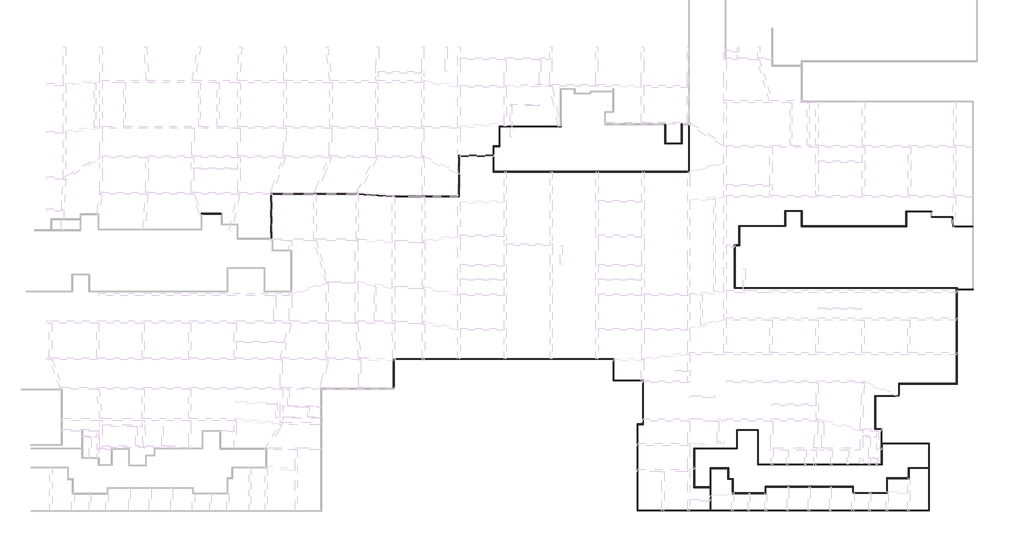
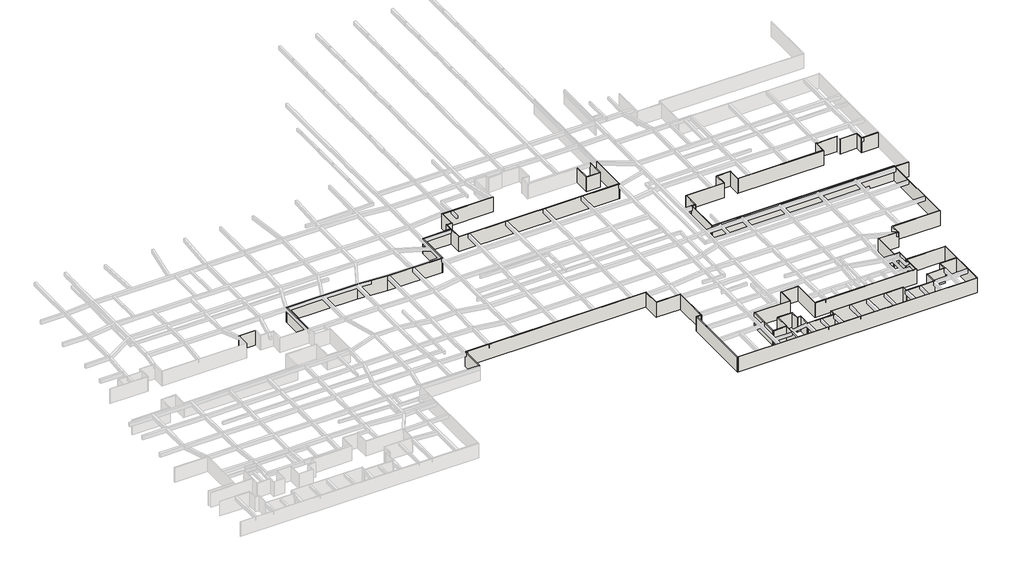
# One storey, part 2 of 16: 71 walls.
"""IFC4 building model written with IfcOpenShell, lengths in millimetres."""

from ifc_helpers import new_model, si_unit, origin, origin_with_axes, place, context, project, spatial, polyline, outline, extrude, faceted_brep, element, save

model = new_model("IFC4")

# Units and contexts
model_context = context("Model", 3, world=origin())
ifc_project = project(units=[si_unit("LENGTHUNIT", "METRE", prefix="MILLI")], contexts=[model_context])

# Site, building, storey
site = spatial("IfcSite", under=ifc_project)
building = spatial("IfcBuilding", under=site)
storey = spatial("IfcBuildingStorey", under=building, Name="户型图", Elevation=0.0)

# Walls
placement = place(None, origin())
element("IfcWall", 1, ObjectType="所有墙体", at=placement, inside=storey, context=model_context, shape_type="Brep", body=[
    faceted_brep([(130041.0654488, 81464.6119076, 0.0), (130041.0654488, 86623.7129117, 0.0), (130041.0654488, 86743.7129117, 0.0), (130041.0654488, 86743.7129117, 3300.0), (130041.0654488, 86623.7129117, 3300.0), (130041.0654488, 81464.6119076, 3300.0), (129921.0654488, 81464.6119076, 0.0), (129921.0654488, 81464.6119076, 3300.0), (129921.0654488, 86743.7129117, 3300.0), (129921.0654488, 86743.7129117, 0.0)], [[[0, 1, 2, 3, 4, 5]], [[6, 7, 8, 9]], [[2, 1, 0, 6, 9]], [[5, 4, 3, 8, 7]], [[0, 5, 7, 6]], [[3, 2, 9, 8]]]),
])
element("IfcWall", 2, ObjectType="所有墙体", at=placement, inside=storey, context=model_context, shape_type="Brep", body=[
    faceted_brep([(130041.0654488, 86623.7129117, 0.0), (168621.0654488, 86623.7129117, 0.0), (168741.0654488, 86623.7129117, 0.0), (168741.0654488, 86623.7129117, 3300.0), (168621.0654488, 86623.7129117, 3300.0), (130041.0654488, 86623.7129117, 3300.0), (130041.0654488, 86743.7129117, 0.0), (130041.0654488, 86743.7129117, 3300.0), (168741.0654488, 86743.7129117, 3300.0), (168741.0654488, 86743.7129117, 0.0)], [[[0, 1, 2, 3, 4, 5]], [[6, 7, 8, 9]], [[2, 1, 0, 6, 9]], [[5, 4, 3, 8, 7]], [[0, 5, 7, 6]], [[3, 2, 9, 8]]]),
])
element("IfcWall", 3, ObjectType="所有墙体", at=placement, inside=storey, context=model_context, shape_type="Brep", body=[
    faceted_brep([(168621.0654488, 86623.7129117, 0.0), (168621.0654488, 82792.1509701, 0.0), (168621.0654488, 82792.1509701, 3300.0), (168621.0654488, 86623.7129117, 3300.0), (168741.0654488, 86623.7129117, 0.0), (168741.0654488, 86623.7129117, 3300.0), (168741.0654488, 82912.1509701, 3300.0), (168741.0654488, 82792.1509701, 3300.0), (168741.0654488, 82792.1509701, 0.0), (168741.0654488, 82912.1509701, 0.0)], [[[0, 1, 2, 3]], [[4, 5, 6, 7, 8, 9]], [[1, 0, 4, 9, 8]], [[3, 2, 7, 6, 5]], [[0, 3, 5, 4]], [[2, 1, 8, 7]]]),
])
element("IfcWall", 4, ObjectType="所有墙体", at=placement, inside=storey, context=model_context, shape_type="Brep", body=[
    faceted_brep([(168741.0654488, 82792.1509701, 0.0), (173812.0751369, 82792.1509701, 0.0), (173932.0751369, 82792.1509701, 0.0), (173932.0751369, 82792.1509701, 3300.0), (173812.0751369, 82792.1509701, 3300.0), (168741.0654488, 82792.1509701, 3300.0), (168741.0654488, 82912.1509701, 0.0), (168741.0654488, 82912.1509701, 3300.0), (173932.0751369, 82912.1509701, 3300.0), (173932.0751369, 82912.1509701, 0.0)], [[[0, 1, 2, 3, 4, 5]], [[6, 7, 8, 9]], [[2, 1, 0, 6, 9]], [[5, 4, 3, 8, 7]], [[0, 5, 7, 6]], [[3, 2, 9, 8]]]),
])
element("IfcWall", 5, ObjectType="所有墙体", at=placement, inside=storey, context=model_context, shape_type="Brep", body=[
    faceted_brep([(173812.0751369, 82792.1509701, 0.0), (173812.0751369, 75212.1509701, 0.0), (173812.0751369, 75092.1509701, 0.0), (173812.0751369, 75092.1509701, 3300.0), (173812.0751369, 75212.1509701, 3300.0), (173812.0751369, 82792.1509701, 3300.0), (173932.0751369, 82792.1509701, 0.0), (173932.0751369, 82792.1509701, 3300.0), (173932.0751369, 75092.1509701, 3300.0), (173932.0751369, 75092.1509701, 0.0)], [[[0, 1, 2, 3, 4, 5]], [[6, 7, 8, 9]], [[2, 1, 0, 6, 9]], [[5, 4, 3, 8, 7]], [[0, 5, 7, 6]], [[3, 2, 9, 8]]]),
])
element("IfcWall", 6, ObjectType="所有墙体", at=placement, inside=storey, context=model_context, shape_type="Brep", body=[
    faceted_brep([(173812.0751369, 75212.1509701, 0.0), (172837.1171537, 75212.1509701, 0.0), (172837.1171537, 75212.1509701, 3300.0), (173812.0751369, 75212.1509701, 3300.0), (173812.0751369, 75092.1509701, 0.0), (173812.0751369, 75092.1509701, 3300.0), (172957.1171537, 75092.1509701, 3300.0), (172837.1171537, 75092.1509701, 3300.0), (172837.1171537, 75092.1509701, 0.0), (172957.1171537, 75092.1509701, 0.0)], [[[0, 1, 2, 3]], [[4, 5, 6, 7, 8, 9]], [[1, 0, 4, 9, 8]], [[3, 2, 7, 6, 5]], [[0, 3, 5, 4]], [[2, 1, 8, 7]]]),
])
element("IfcWall", 7, ObjectType="所有墙体", at=placement, inside=storey, context=model_context, shape_type="Brep", body=[
    faceted_brep([(172837.1171537, 75092.1509701, 0.0), (172837.1171537, 59892.1509701, 0.0), (172837.1171537, 59892.1509701, 3300.0), (172837.1171537, 75092.1509701, 3300.0), (172957.1171537, 75092.1509701, 0.0), (172957.1171537, 75092.1509701, 3300.0), (172957.1171537, 60012.1509701, 3300.0), (172957.1171537, 59892.1509701, 3300.0), (172957.1171537, 59892.1509701, 0.0), (172957.1171537, 60012.1509701, 0.0)], [[[0, 1, 2, 3]], [[4, 5, 6, 7, 8, 9]], [[1, 0, 4, 9, 8]], [[3, 2, 7, 6, 5]], [[0, 3, 5, 4]], [[2, 1, 8, 7]]]),
])
element("IfcWall", 8, ObjectType="所有墙体", at=placement, inside=storey, context=model_context, shape_type="Brep", body=[
    faceted_brep([(172957.1171537, 59892.1509701, 0.0), (224357.1171537, 59892.1509701, 0.0), (224357.1171537, 59892.1509701, 3300.0), (172957.1171537, 59892.1509701, 3300.0), (172957.1171537, 60012.1509701, 0.0), (172957.1171537, 60012.1509701, 3300.0), (185686.7118802, 60012.1509701, 3300.0), (185806.7118802, 60012.1509701, 3300.0), (224237.1171537, 60012.1509701, 3300.0), (224357.1171537, 60012.1509701, 3300.0), (224357.1171537, 60012.1509701, 0.0), (224237.1171537, 60012.1509701, 0.0), (185806.7118802, 60012.1509701, 0.0), (185686.7118802, 60012.1509701, 0.0)], [[[0, 1, 2, 3]], [[4, 5, 6, 7, 8, 9, 10, 11, 12, 13]], [[1, 0, 4, 13, 12, 11, 10]], [[3, 2, 9, 8, 7, 6, 5]], [[0, 3, 5, 4]], [[2, 1, 10, 9]]]),
])
element("IfcWall", 9, ObjectType="所有墙体", at=placement, inside=storey, context=model_context, shape_type="Brep", body=[
    faceted_brep([(224357.1171537, 60012.1509701, 0.0), (224357.1171537, 71812.1509701, 0.0), (224357.1171537, 71812.1509701, 3300.0), (224357.1171537, 60012.1509701, 3300.0), (224237.1171537, 60012.1509701, 0.0), (224237.1171537, 60012.1509701, 3300.0), (224237.1171537, 67402.3902279, 3300.0), (224237.1171537, 67522.3902279, 3300.0), (224237.1171537, 71692.1509701, 3300.0), (224237.1171537, 71812.1509701, 3300.0), (224237.1171537, 71812.1509701, 0.0), (224237.1171537, 71692.1509701, 0.0), (224237.1171537, 67522.3902279, 0.0), (224237.1171537, 67402.3902279, 0.0)], [[[0, 1, 2, 3]], [[4, 5, 6, 7, 8, 9, 10, 11, 12, 13]], [[1, 0, 4, 13, 12, 11, 10]], [[3, 2, 9, 8, 7, 6, 5]], [[0, 3, 5, 4]], [[2, 1, 10, 9]]]),
])
element("IfcWall", 10, ObjectType="所有墙体", at=placement, inside=storey, context=model_context, shape_type="Brep", body=[
    faceted_brep([(224237.1171537, 71812.1509701, 0.0), (215957.1171537, 71812.1509701, 0.0), (215837.1171537, 71812.1509701, 0.0), (215837.1171537, 71812.1509701, 3300.0), (215957.1171537, 71812.1509701, 3300.0), (224237.1171537, 71812.1509701, 3300.0), (224237.1171537, 71692.1509701, 0.0), (224237.1171537, 71692.1509701, 3300.0), (216006.7104154, 71692.1509701, 3300.0), (215886.7104154, 71692.1509701, 3300.0), (215837.1171537, 71692.1509701, 3300.0), (215837.1171537, 71692.1509701, 0.0), (215886.7104154, 71692.1509701, 0.0), (216006.7104154, 71692.1509701, 0.0)], [[[0, 1, 2, 3, 4, 5]], [[6, 7, 8, 9, 10, 11, 12, 13]], [[2, 1, 0, 6, 13, 12, 11]], [[5, 4, 3, 10, 9, 8, 7]], [[0, 5, 7, 6]], [[3, 2, 11, 10]]]),
])
element("IfcWall", 11, ObjectType="所有墙体", at=placement, inside=storey, context=model_context, shape_type="Brep", body=[
    faceted_brep([(215957.1171537, 71812.1509701, 0.0), (215957.1171537, 74372.3072201, 0.0), (215957.1171537, 74372.3072201, 3300.0), (215957.1171537, 71812.1509701, 3300.0), (215837.1171537, 71812.1509701, 0.0), (215837.1171537, 71812.1509701, 3300.0), (215837.1171537, 74252.3072201, 3300.0), (215837.1171537, 74372.3072201, 3300.0), (215837.1171537, 74372.3072201, 0.0), (215837.1171537, 74252.3072201, 0.0)], [[[0, 1, 2, 3]], [[4, 5, 6, 7, 8, 9]], [[1, 0, 4, 9, 8]], [[3, 2, 7, 6, 5]], [[0, 3, 5, 4]], [[2, 1, 8, 7]]]),
])
element("IfcWall", 12, ObjectType="所有墙体", at=placement, inside=storey, context=model_context, shape_type="Brep", body=[
    faceted_brep([(215837.1171537, 74372.3072201, 0.0), (214857.1171537, 74372.3072201, 0.0), (214737.1171537, 74372.3072201, 0.0), (214737.1171537, 74372.3072201, 3300.0), (214857.1171537, 74372.3072201, 3300.0), (215837.1171537, 74372.3072201, 3300.0), (215837.1171537, 74252.3072201, 0.0), (215837.1171537, 74252.3072201, 3300.0), (214737.1171537, 74252.3072201, 3300.0), (214737.1171537, 74252.3072201, 0.0)], [[[0, 1, 2, 3, 4, 5]], [[6, 7, 8, 9]], [[2, 1, 0, 6, 9]], [[5, 4, 3, 8, 7]], [[0, 5, 7, 6]], [[3, 2, 9, 8]]]),
])
element("IfcWall", 13, ObjectType="所有墙体", at=placement, inside=storey, context=model_context, shape_type="Brep", body=[
    faceted_brep([(214857.1171537, 74372.3072201, 0.0), (214857.1171537, 80052.3072201, 0.0), (214857.1171537, 80172.3072201, 0.0), (214857.1171537, 80172.3072201, 3300.0), (214857.1171537, 80052.3072201, 3300.0), (214857.1171537, 74372.3072201, 3300.0), (214737.1171537, 74372.3072201, 0.0), (214737.1171537, 74372.3072201, 3300.0), (214737.1171537, 80172.3072201, 3300.0), (214737.1171537, 80172.3072201, 0.0)], [[[0, 1, 2, 3, 4, 5]], [[6, 7, 8, 9]], [[2, 1, 0, 6, 9]], [[5, 4, 3, 8, 7]], [[0, 5, 7, 6]], [[3, 2, 9, 8]]]),
])
element("IfcWall", 14, ObjectType="所有墙体", at=placement, inside=storey, context=model_context, shape_type="Brep", body=[
    faceted_brep([(214857.1171537, 80052.3072201, 0.0), (219065.7473941, 80052.3072201, 0.0), (219065.7473941, 80052.3072201, 3300.0), (214857.1171537, 80052.3072201, 3300.0), (214857.1171537, 80172.3072201, 0.0), (214857.1171537, 80172.3072201, 3300.0), (218945.7473941, 80172.3072201, 3300.0), (219065.7473941, 80172.3072201, 3300.0), (219065.7473941, 80172.3072201, 0.0), (218945.7473941, 80172.3072201, 0.0)], [[[0, 1, 2, 3]], [[4, 5, 6, 7, 8, 9]], [[1, 0, 4, 9, 8]], [[3, 2, 7, 6, 5]], [[0, 3, 5, 4]], [[2, 1, 8, 7]]]),
])
element("IfcWall", 15, ObjectType="所有墙体", at=placement, inside=storey, context=model_context, shape_type="Brep", body=[
    faceted_brep([(219065.7473941, 80172.3072201, 0.0), (219065.7473941, 82242.2134701, 0.0), (219065.7473941, 82362.2134701, 0.0), (219065.7473941, 82362.2134701, 3300.0), (219065.7473941, 82242.2134701, 3300.0), (219065.7473941, 80172.3072201, 3300.0), (218945.7473941, 80172.3072201, 0.0), (218945.7473941, 80172.3072201, 3300.0), (218945.7473941, 82362.2134701, 3300.0), (218945.7473941, 82362.2134701, 0.0)], [[[0, 1, 2, 3, 4, 5]], [[6, 7, 8, 9]], [[2, 1, 0, 6, 9]], [[5, 4, 3, 8, 7]], [[0, 5, 7, 6]], [[3, 2, 9, 8]]]),
])
element("IfcWall", 16, ObjectType="所有墙体", at=placement, inside=storey, context=model_context, shape_type="Brep", body=[
    faceted_brep([(219065.7473941, 82242.2134701, 0.0), (229226.2421537, 82242.2134701, 0.0), (229226.2421537, 82242.2134701, 3300.0), (219065.7473941, 82242.2134701, 3300.0), (219065.7473941, 82362.2134701, 0.0), (219065.7473941, 82362.2134701, 3300.0), (229106.2421537, 82362.2134701, 3300.0), (229226.2421537, 82362.2134701, 3300.0), (229226.2421537, 82362.2134701, 0.0), (229106.2421537, 82362.2134701, 0.0)], [[[0, 1, 2, 3]], [[4, 5, 6, 7, 8, 9]], [[1, 0, 4, 9, 8]], [[3, 2, 7, 6, 5]], [[0, 3, 5, 4]], [[2, 1, 8, 7]]]),
])
element("IfcWall", 17, ObjectType="所有墙体", at=placement, inside=storey, context=model_context, shape_type="Brep", body=[
    faceted_brep([(229226.2421537, 82362.2134701, 0.0), (229226.2421537, 98851.3072201, 0.0), (229226.2421537, 98971.3072201, 0.0), (229226.2421537, 99221.2967221, 0.0), (229226.2421537, 99221.2967221, 3300.0), (229226.2421537, 98971.3072201, 3300.0), (229226.2421537, 98851.3072201, 3300.0), (229226.2421537, 82362.2134701, 3300.0), (229106.2421537, 82362.2134701, 0.0), (229106.2421537, 82362.2134701, 3300.0), (229106.2421537, 99101.2967221, 3300.0), (229106.2421537, 99221.2967221, 3300.0), (229106.2421537, 99221.2967221, 0.0), (229106.2421537, 99101.2967221, 0.0)], [[[0, 1, 2, 3, 4, 5, 6, 7]], [[8, 9, 10, 11, 12, 13]], [[3, 2, 1, 0, 8, 13, 12]], [[7, 6, 5, 4, 11, 10, 9]], [[0, 7, 9, 8]], [[4, 3, 12, 11]]]),
])
element("IfcWall", 18, ObjectType="所有墙体", at=placement, inside=storey, context=model_context, shape_type="Brep", body=[
    faceted_brep([(229226.2421537, 98851.3072201, 0.0), (232107.9308744, 98851.3072201, 0.0), (232107.9308744, 98851.3072201, 3300.0), (229226.2421537, 98851.3072201, 3300.0), (229226.2421537, 98971.3072201, 0.0), (229226.2421537, 98971.3072201, 3300.0), (231987.9308744, 98971.3072201, 3300.0), (232107.9308744, 98971.3072201, 3300.0), (232107.9308744, 98971.3072201, 0.0), (231987.9308744, 98971.3072201, 0.0)], [[[0, 1, 2, 3]], [[4, 5, 6, 7, 8, 9]], [[1, 0, 4, 9, 8]], [[3, 2, 7, 6, 5]], [[2, 1, 8, 7]], [[0, 3, 5, 4]]]),
])
element("IfcWall", 19, ObjectType="所有墙体", at=placement, inside=storey, context=model_context, shape_type="Brep", body=[
    faceted_brep([(99612.3510404, 112314.5259701, 0.0), (96012.3510404, 112314.5259701, 0.0), (96012.3510404, 112314.5259701, 3300.0), (99612.3510404, 112314.5259701, 3300.0), (99612.3510404, 112194.5259701, 0.0), (99612.3510404, 112194.5259701, 3300.0), (96132.3510404, 112194.5259701, 3300.0), (96012.3510404, 112194.5259701, 3300.0), (96012.3510404, 112194.5259701, 0.0), (96132.3510404, 112194.5259701, 0.0)], [[[0, 1, 2, 3]], [[4, 5, 6, 7, 8, 9]], [[1, 0, 4, 9, 8]], [[3, 2, 7, 6, 5]], [[0, 3, 5, 4]], [[2, 1, 8, 7]]]),
])
element("IfcWall", 20, ObjectType="所有墙体", at=placement, inside=storey, context=model_context, shape_type="Brep", body=[
    faceted_brep([(177743.2890287, 127952.5884701, 0.0), (177743.2890287, 124552.5884701, 0.0), (177743.2890287, 124552.5884701, 3300.0), (177743.2890287, 127952.5884701, 3300.0), (177863.2890287, 127952.5884701, 0.0), (177863.2890287, 127952.5884701, 3300.0), (177863.2890287, 124672.5884701, 3300.0), (177863.2890287, 124552.5884701, 3300.0), (177863.2890287, 124552.5884701, 0.0), (177863.2890287, 124672.5884701, 0.0)], [[[0, 1, 2, 3]], [[4, 5, 6, 7, 8, 9]], [[1, 0, 4, 9, 8]], [[3, 2, 7, 6, 5]], [[0, 3, 5, 4]], [[2, 1, 8, 7]]]),
])
element("IfcWall", 21, ObjectType="所有墙体", at=placement, inside=storey, context=model_context, shape_type="Brep", body=[
    faceted_brep([(177863.2890287, 124552.5884701, 0.0), (180763.3460986, 124552.5884701, 0.0), (180763.3460986, 124552.5884701, 3300.0), (177863.2890287, 124552.5884701, 3300.0), (177863.2890287, 124672.5884701, 0.0), (177863.2890287, 124672.5884701, 3300.0), (180643.3460986, 124672.5884701, 3300.0), (180763.3460986, 124672.5884701, 3300.0), (180763.3460986, 124672.5884701, 0.0), (180643.3460986, 124672.5884701, 0.0)], [[[0, 1, 2, 3]], [[4, 5, 6, 7, 8, 9]], [[1, 0, 4, 9, 8]], [[3, 2, 7, 6, 5]], [[0, 3, 5, 4]], [[2, 1, 8, 7]]]),
])
element("IfcWall", 22, ObjectType="所有墙体", at=placement, inside=storey, context=model_context, shape_type="Brep", body=[
    faceted_brep([(180763.3460986, 124672.5884701, 0.0), (180763.3460986, 127952.5884701, 0.0), (180763.3460986, 128072.5884701, 0.0), (180763.3460986, 128072.5884701, 3300.0), (180763.3460986, 127952.5884701, 3300.0), (180763.3460986, 124672.5884701, 3300.0), (180643.3460986, 124672.5884701, 0.0), (180643.3460986, 124672.5884701, 3300.0), (180643.3460986, 128072.5884701, 3300.0), (180643.3460986, 128072.5884701, 0.0)], [[[0, 1, 2, 3, 4, 5]], [[6, 7, 8, 9]], [[2, 1, 0, 6, 9]], [[5, 4, 3, 8, 7]], [[0, 5, 7, 6]], [[3, 2, 9, 8]]]),
])
element("IfcWall", 23, ObjectType="所有墙体", at=placement, inside=storey, context=model_context, shape_type="Brep", body=[
    faceted_brep([(181897.7367524, 127952.5884701, 0.0), (181897.7367524, 119698.0259701, 0.0), (181897.7367524, 119578.0259701, 0.0), (181897.7367524, 119578.0259701, 3300.0), (181897.7367524, 119698.0259701, 3300.0), (181897.7367524, 127952.5884701, 3300.0), (182017.7367524, 127952.5884701, 0.0), (182017.7367524, 127952.5884701, 3300.0), (182017.7367524, 119578.0259701, 3300.0), (182017.7367524, 119578.0259701, 0.0)], [[[0, 1, 2, 3, 4, 5]], [[6, 7, 8, 9]], [[2, 1, 0, 6, 9]], [[5, 4, 3, 8, 7]], [[3, 2, 9, 8]], [[0, 5, 7, 6]]]),
])
element("IfcWall", 24, ObjectType="所有墙体", at=placement, inside=storey, context=model_context, shape_type="Brep", body=[
    faceted_brep([(181897.7367524, 119698.0259701, 0.0), (147617.7367524, 119698.0259701, 0.0), (147497.7367524, 119698.0259701, 0.0), (147497.7367524, 119698.0259701, 3300.0), (147617.7367524, 119698.0259701, 3300.0), (181897.7367524, 119698.0259701, 3300.0), (181897.7367524, 119578.0259701, 0.0), (181897.7367524, 119578.0259701, 3300.0), (147497.7367524, 119578.0259701, 3300.0), (147497.7367524, 119578.0259701, 0.0)], [[[0, 1, 2, 3, 4, 5]], [[6, 7, 8, 9]], [[2, 1, 0, 6, 9]], [[5, 4, 3, 8, 7]], [[0, 5, 7, 6]], [[3, 2, 9, 8]]]),
])
element("IfcWall", 25, ObjectType="所有墙体", at=placement, inside=storey, context=model_context, shape_type="Brep", body=[
    faceted_brep([(147617.7367524, 119698.0259701, 0.0), (147617.7367524, 124078.0259701, 0.0), (147617.7367524, 124198.0259701, 0.0), (147617.7367524, 124198.0259701, 3300.0), (147617.7367524, 124078.0259701, 3300.0), (147617.7367524, 119698.0259701, 3300.0), (147497.7367524, 119698.0259701, 0.0), (147497.7367524, 119698.0259701, 3300.0), (147497.7367524, 122418.0259701, 3300.0), (147497.7367524, 122538.0259701, 3300.0), (147497.7367524, 124198.0259701, 3300.0), (147497.7367524, 124198.0259701, 0.0), (147497.7367524, 122538.0259701, 0.0), (147497.7367524, 122418.0259701, 0.0)], [[[0, 1, 2, 3, 4, 5]], [[6, 7, 8, 9, 10, 11, 12, 13]], [[2, 1, 0, 6, 13, 12, 11]], [[5, 4, 3, 10, 9, 8, 7]], [[0, 5, 7, 6]], [[3, 2, 11, 10]]]),
])
element("IfcWall", 26, ObjectType="所有墙体", at=placement, inside=storey, context=model_context, shape_type="Brep", body=[
    faceted_brep([(147617.7367524, 124078.0259701, 0.0), (148663.2890287, 124078.0259701, 0.0), (148663.2890287, 124078.0259701, 3300.0), (147617.7367524, 124078.0259701, 3300.0), (147617.7367524, 124198.0259701, 0.0), (147617.7367524, 124198.0259701, 3300.0), (148543.2890287, 124198.0259701, 3300.0), (148663.2890287, 124198.0259701, 3300.0), (148663.2890287, 124198.0259701, 0.0), (148543.2890287, 124198.0259701, 0.0)], [[[0, 1, 2, 3]], [[4, 5, 6, 7, 8, 9]], [[1, 0, 4, 9, 8]], [[3, 2, 7, 6, 5]], [[0, 3, 5, 4]], [[2, 1, 8, 7]]]),
])
element("IfcWall", 27, ObjectType="所有墙体", at=placement, inside=storey, context=model_context, shape_type="Brep", body=[
    faceted_brep([(148663.2890287, 124198.0259701, 0.0), (148663.2890287, 127578.0259701, 0.0), (148663.2890287, 127698.0259701, 0.0), (148663.2890287, 127698.0259701, 3300.0), (148663.2890287, 127578.0259701, 3300.0), (148663.2890287, 124198.0259701, 3300.0), (148543.2890287, 124198.0259701, 0.0), (148543.2890287, 124198.0259701, 3300.0), (148543.2890287, 127698.0259701, 3300.0), (148543.2890287, 127698.0259701, 0.0)], [[[0, 1, 2, 3, 4, 5]], [[6, 7, 8, 9]], [[2, 1, 0, 6, 9]], [[5, 4, 3, 8, 7]], [[0, 5, 7, 6]], [[3, 2, 9, 8]]]),
])
element("IfcWall", 28, ObjectType="所有墙体", at=placement, inside=storey, context=model_context, shape_type="Brep", body=[
    faceted_brep([(148663.2890287, 127578.0259701, 0.0), (159463.2890287, 127578.0259701, 0.0), (159463.2890287, 127578.0259701, 3300.0), (148663.2890287, 127578.0259701, 3300.0), (148663.2890287, 127698.0259701, 0.0), (148663.2890287, 127698.0259701, 3300.0), (159343.2890287, 127698.0259701, 3300.0), (159463.2890287, 127698.0259701, 3300.0), (159463.2890287, 127698.0259701, 0.0), (159343.2890287, 127698.0259701, 0.0)], [[[0, 1, 2, 3]], [[4, 5, 6, 7, 8, 9]], [[1, 0, 4, 9, 8]], [[3, 2, 7, 6, 5]], [[0, 3, 5, 4]], [[2, 1, 8, 7]]]),
])
element("IfcWall", 29, ObjectType="所有墙体", at=placement, inside=storey, context=model_context, shape_type="Brep", body=[
    faceted_brep([(199007.9283109, 110171.2134701, 0.0), (198887.9283109, 110171.2134701, 0.0), (190787.9283109, 110171.2134701, 0.0), (190787.9283109, 110171.2134701, 3300.0), (198887.9283109, 110171.2134701, 3300.0), (199007.9283109, 110171.2134701, 3300.0), (199007.9283109, 110051.2134701, 0.0), (199007.9283109, 110051.2134701, 3300.0), (190907.9283109, 110051.2134701, 3300.0), (190787.9283109, 110051.2134701, 3300.0), (190787.9283109, 110051.2134701, 0.0), (190907.9283109, 110051.2134701, 0.0)], [[[0, 1, 2, 3, 4, 5]], [[6, 7, 8, 9, 10, 11]], [[2, 1, 0, 6, 11, 10]], [[5, 4, 3, 9, 8, 7]], [[3, 2, 10, 9]], [[0, 5, 7, 6]]]),
])
element("IfcWall", 30, ObjectType="所有墙体", at=placement, inside=storey, context=model_context, shape_type="Brep", body=[
    faceted_brep([(190787.9283109, 110051.2134701, 0.0), (190787.9283109, 106771.2090896, 0.0), (190787.9283109, 106651.2090896, 0.0), (190787.9283109, 106651.2090896, 3300.0), (190787.9283109, 106771.2090896, 3300.0), (190787.9283109, 110051.2134701, 3300.0), (190907.9283109, 110051.2134701, 0.0), (190907.9283109, 110051.2134701, 3300.0), (190907.9283109, 106651.2090896, 3300.0), (190907.9283109, 106651.2090896, 0.0)], [[[0, 1, 2, 3, 4, 5]], [[6, 7, 8, 9]], [[2, 1, 0, 6, 9]], [[5, 4, 3, 8, 7]], [[0, 5, 7, 6]], [[3, 2, 9, 8]]]),
])
element("IfcWall", 31, ObjectType="所有墙体", at=placement, inside=storey, context=model_context, shape_type="Brep", body=[
    faceted_brep([(190787.9283109, 106771.2090896, 0.0), (189987.9283109, 106771.2090896, 0.0), (189987.9283109, 106771.2090896, 3300.0), (190787.9283109, 106771.2090896, 3300.0), (190787.9283109, 106651.2090896, 0.0), (190787.9283109, 106651.2090896, 3300.0), (190107.9283109, 106651.2090896, 3300.0), (189987.9283109, 106651.2090896, 3300.0), (189987.9283109, 106651.2090896, 0.0), (190107.9283109, 106651.2090896, 0.0)], [[[0, 1, 2, 3]], [[4, 5, 6, 7, 8, 9]], [[1, 0, 4, 9, 8]], [[3, 2, 7, 6, 5]], [[0, 3, 5, 4]], [[2, 1, 8, 7]]]),
])
element("IfcWall", 32, ObjectType="所有墙体", at=placement, inside=storey, context=model_context, shape_type="Brep", body=[
    faceted_brep([(189987.9283109, 106651.2090896, 0.0), (189987.9283109, 99101.2967221, 0.0), (189987.9283109, 99101.2967221, 3300.0), (189987.9283109, 106651.2090896, 3300.0), (190107.9283109, 106651.2090896, 0.0), (190107.9283109, 106651.2090896, 3300.0), (190107.9283109, 99221.2967221, 3300.0), (190107.9283109, 99101.2967221, 3300.0), (190107.9283109, 99101.2967221, 0.0), (190107.9283109, 99221.2967221, 0.0)], [[[0, 1, 2, 3]], [[4, 5, 6, 7, 8, 9]], [[1, 0, 4, 9, 8]], [[3, 2, 7, 6, 5]], [[0, 3, 5, 4]], [[2, 1, 8, 7]]]),
])
element("IfcWall", 33, ObjectType="所有墙体", at=placement, inside=storey, context=model_context, shape_type="SweptSolid", body=[
    extrude(outline(polyline([(190107.9283109, 99221.2967221), (229106.2421537, 99221.2967221), (229106.2421537, 99101.2967221), (190107.9283109, 99101.2967221), (190107.9283109, 99221.2967221)])), origin_with_axes(), (0.0, 0.0, 1.0), 3300.0),
])
element("IfcWall", 34, ObjectType="所有墙体", at=placement, inside=storey, context=model_context, shape_type="Brep", body=[
    faceted_brep([(199007.9283109, 110171.2134701, 0.0), (199007.9283109, 112701.2124935, 0.0), (199007.9283109, 112821.2124935, 0.0), (199007.9283109, 112821.2124935, 3300.0), (199007.9283109, 112701.2124935, 3300.0), (199007.9283109, 110171.2134701, 3300.0), (198887.9283109, 110171.2134701, 0.0), (198887.9283109, 110171.2134701, 3300.0), (198887.9283109, 112821.2124935, 3300.0), (198887.9283109, 112821.2124935, 0.0)], [[[0, 1, 2, 3, 4, 5]], [[6, 7, 8, 9]], [[2, 1, 0, 6, 9]], [[5, 4, 3, 8, 7]], [[0, 5, 7, 6]], [[3, 2, 9, 8]]]),
])
element("IfcWall", 35, ObjectType="所有墙体", at=placement, inside=storey, context=model_context, shape_type="Brep", body=[
    faceted_brep([(199007.9283109, 112701.2124935, 0.0), (201787.9283109, 112701.2124935, 0.0), (201907.9283109, 112701.2124935, 0.0), (201907.9283109, 112701.2124935, 3300.0), (201787.9283109, 112701.2124935, 3300.0), (199007.9283109, 112701.2124935, 3300.0), (199007.9283109, 112821.2124935, 0.0), (199007.9283109, 112821.2124935, 3300.0), (201907.9283109, 112821.2124935, 3300.0), (201907.9283109, 112821.2124935, 0.0)], [[[0, 1, 2, 3, 4, 5]], [[6, 7, 8, 9]], [[2, 1, 0, 6, 9]], [[5, 4, 3, 8, 7]], [[0, 5, 7, 6]], [[3, 2, 9, 8]]]),
])
element("IfcWall", 36, ObjectType="所有墙体", at=placement, inside=storey, context=model_context, shape_type="Brep", body=[
    faceted_brep([(201787.9283109, 112701.2124935, 0.0), (201787.9283109, 110001.2124935, 0.0), (201787.9283109, 110001.2124935, 3300.0), (201787.9283109, 112701.2124935, 3300.0), (201907.9283109, 112701.2124935, 0.0), (201907.9283109, 112701.2124935, 3300.0), (201907.9283109, 110121.2124935, 3300.0), (201907.9283109, 110001.2124935, 3300.0), (201907.9283109, 110001.2124935, 0.0), (201907.9283109, 110121.2124935, 0.0)], [[[0, 1, 2, 3]], [[4, 5, 6, 7, 8, 9]], [[1, 0, 4, 9, 8]], [[3, 2, 7, 6, 5]], [[0, 3, 5, 4]], [[2, 1, 8, 7]]]),
])
element("IfcWall", 37, ObjectType="所有墙体", at=placement, inside=storey, context=model_context, shape_type="Brep", body=[
    faceted_brep([(201907.9283109, 110001.2124935, 0.0), (220307.9283109, 110001.2124935, 0.0), (220307.9283109, 110001.2124935, 3300.0), (201907.9283109, 110001.2124935, 3300.0), (201907.9283109, 110121.2124935, 0.0), (201907.9283109, 110121.2124935, 3300.0), (220187.9283109, 110121.2124935, 3300.0), (220307.9283109, 110121.2124935, 3300.0), (220307.9283109, 110121.2124935, 0.0), (220187.9283109, 110121.2124935, 0.0)], [[[0, 1, 2, 3]], [[4, 5, 6, 7, 8, 9]], [[1, 0, 4, 9, 8]], [[3, 2, 7, 6, 5]], [[0, 3, 5, 4]], [[2, 1, 8, 7]]]),
])
element("IfcWall", 38, ObjectType="所有墙体", at=placement, inside=storey, context=model_context, shape_type="Brep", body=[
    faceted_brep([(220307.9283109, 110121.2124935, 0.0), (220307.9283109, 112601.2124935, 0.0), (220307.9283109, 112721.2124935, 0.0), (220307.9283109, 112721.2124935, 3300.0), (220307.9283109, 112601.2124935, 3300.0), (220307.9283109, 110121.2124935, 3300.0), (220187.9283109, 110121.2124935, 0.0), (220187.9283109, 110121.2124935, 3300.0), (220187.9283109, 112721.2124935, 3300.0), (220187.9283109, 112721.2124935, 0.0)], [[[0, 1, 2, 3, 4, 5]], [[6, 7, 8, 9]], [[2, 1, 0, 6, 9]], [[5, 4, 3, 8, 7]], [[0, 5, 7, 6]], [[3, 2, 9, 8]]]),
])
element("IfcWall", 39, ObjectType="所有墙体", at=placement, inside=storey, context=model_context, shape_type="Brep", body=[
    faceted_brep([(220307.9283109, 112601.2124935, 0.0), (224612.920801, 112601.2124935, 0.0), (224732.920801, 112601.2124935, 0.0), (224732.920801, 112601.2124935, 3300.0), (224612.920801, 112601.2124935, 3300.0), (220307.9283109, 112601.2124935, 3300.0), (220307.9283109, 112721.2124935, 0.0), (220307.9283109, 112721.2124935, 3300.0), (224732.920801, 112721.2124935, 3300.0), (224732.920801, 112721.2124935, 0.0)], [[[0, 1, 2, 3, 4, 5]], [[6, 7, 8, 9]], [[2, 1, 0, 6, 9]], [[5, 4, 3, 8, 7]], [[0, 5, 7, 6]], [[3, 2, 9, 8]]]),
])
element("IfcWall", 40, ObjectType="所有墙体", at=placement, inside=storey, context=model_context, shape_type="Brep", body=[
    faceted_brep([(224732.920801, 111591.2134701, 0.0), (228339.2678157, 111591.2134701, 0.0), (228459.2678157, 111591.2134701, 0.0), (228459.2678157, 111591.2134701, 3300.0), (228339.2678157, 111591.2134701, 3300.0), (224732.920801, 111591.2134701, 3300.0), (224732.920801, 111711.2134701, 0.0), (224732.920801, 111711.2134701, 3300.0), (228459.2678157, 111711.2134701, 3300.0), (228459.2678157, 111711.2134701, 0.0)], [[[0, 1, 2, 3, 4, 5]], [[6, 7, 8, 9]], [[2, 1, 0, 6, 9]], [[5, 4, 3, 8, 7]], [[0, 5, 7, 6]], [[3, 2, 9, 8]]]),
])
element("IfcWall", 41, ObjectType="所有墙体", at=placement, inside=storey, context=model_context, shape_type="Brep", body=[
    faceted_brep([(228339.2678157, 111591.2134701, 0.0), (228339.2678157, 109971.2134701, 0.0), (228339.2678157, 109971.2134701, 3300.0), (228339.2678157, 111591.2134701, 3300.0), (228459.2678157, 111591.2134701, 0.0), (228459.2678157, 111591.2134701, 3300.0), (228459.2678157, 110091.2134701, 3300.0), (228459.2678157, 109971.2134701, 3300.0), (228459.2678157, 109971.2134701, 0.0), (228459.2678157, 110091.2134701, 0.0)], [[[0, 1, 2, 3]], [[4, 5, 6, 7, 8, 9]], [[1, 0, 4, 9, 8]], [[3, 2, 7, 6, 5]], [[0, 3, 5, 4]], [[2, 1, 8, 7]]]),
])
element("IfcWall", 42, ObjectType="所有墙体", at=placement, inside=storey, context=model_context, shape_type="SweptSolid", body=[
    extrude(outline(polyline([(231987.9308744, 109971.2134701), (228459.2678157, 109971.2134701), (228459.2678157, 110091.2134701), (231987.9308744, 110091.2134701), (231987.9308744, 109971.2134701)])), origin_with_axes(), (0.0, 0.0, 1.0), 3300.0),
])
element("IfcWall", 43, ObjectType="所有墙体", at=placement, inside=storey, context=model_context, shape_type="Brep", body=[
    faceted_brep([(182836.7178046, 70922.3072201, 0.0), (182836.7178046, 64002.3072201, 0.0), (182836.7178046, 64002.3072201, 3300.0), (182836.7178046, 70922.3072201, 3300.0), (182956.7178046, 70922.3072201, 0.0), (182956.7178046, 70922.3072201, 3300.0), (182956.7178046, 70802.3072201, 3300.0), (182956.7178046, 64122.3072201, 3300.0), (182956.7178046, 64002.3072201, 3300.0), (182956.7178046, 64002.3072201, 0.0), (182956.7178046, 64122.3072201, 0.0), (182956.7178046, 70802.3072201, 0.0)], [[[0, 1, 2, 3]], [[4, 5, 6, 7, 8, 9, 10, 11]], [[1, 0, 4, 11, 10, 9]], [[3, 2, 8, 7, 6, 5]], [[2, 1, 9, 8]], [[0, 3, 5, 4]]]),
])
element("IfcWall", 44, ObjectType="所有墙体", at=placement, inside=storey, context=model_context, shape_type="Brep", body=[
    faceted_brep([(182956.7178046, 64002.3072201, 0.0), (185686.7118802, 64002.3072201, 0.0), (185806.7118802, 64002.3072201, 0.0), (185806.7118802, 64002.3072201, 3300.0), (185686.7118802, 64002.3072201, 3300.0), (182956.7178046, 64002.3072201, 3300.0), (182956.7178046, 64122.3072201, 0.0), (182956.7178046, 64122.3072201, 3300.0), (185736.7118802, 64122.3072201, 3300.0), (185806.7118802, 64122.3072201, 3300.0), (185806.7118802, 64122.3072201, 0.0), (185736.7118802, 64122.3072201, 0.0)], [[[0, 1, 2, 3, 4, 5]], [[6, 7, 8, 9, 10, 11]], [[2, 1, 0, 6, 11, 10]], [[5, 4, 3, 9, 8, 7]], [[0, 5, 7, 6]], [[3, 2, 10, 9]]]),
])
element("IfcWall", 45, ObjectType="所有墙体", at=placement, inside=storey, context=model_context, shape_type="SweptSolid", body=[
    extrude(outline(polyline([(185686.7118802, 60012.1509701), (185686.7118802, 64002.3072201), (185806.7118802, 64002.3072201), (185806.7118802, 60012.1509701), (185686.7118802, 60012.1509701)])), origin_with_axes(), (0.0, 0.0, 1.0), 3300.0),
])
element("IfcWall", 46, ObjectType="所有墙体", at=placement, inside=storey, context=model_context, shape_type="Brep", body=[
    faceted_brep([(182956.7178046, 70802.3072201, 0.0), (190506.7104154, 70802.3072201, 0.0), (190506.7104154, 70802.3072201, 3300.0), (182956.7178046, 70802.3072201, 3300.0), (182956.7178046, 70922.3072201, 0.0), (182956.7178046, 70922.3072201, 3300.0), (190386.7104154, 70922.3072201, 3300.0), (190506.7104154, 70922.3072201, 3300.0), (190506.7104154, 70922.3072201, 0.0), (190386.7104154, 70922.3072201, 0.0)], [[[0, 1, 2, 3]], [[4, 5, 6, 7, 8, 9]], [[1, 0, 4, 9, 8]], [[3, 2, 7, 6, 5]], [[0, 3, 5, 4]], [[2, 1, 8, 7]]]),
])
element("IfcWall", 47, ObjectType="所有墙体", at=placement, inside=storey, context=model_context, shape_type="Brep", body=[
    faceted_brep([(190506.7104154, 70922.3072201, 0.0), (190506.7104154, 74102.3072201, 0.0), (190506.7104154, 74222.3072201, 0.0), (190506.7104154, 74222.3072201, 3300.0), (190506.7104154, 74102.3072201, 3300.0), (190506.7104154, 70922.3072201, 3300.0), (190386.7104154, 70922.3072201, 0.0), (190386.7104154, 70922.3072201, 3300.0), (190386.7104154, 74222.3072201, 3300.0), (190386.7104154, 74222.3072201, 0.0)], [[[0, 1, 2, 3, 4, 5]], [[6, 7, 8, 9]], [[2, 1, 0, 6, 9]], [[5, 4, 3, 8, 7]], [[0, 5, 7, 6]], [[3, 2, 9, 8]]]),
])
element("IfcWall", 48, ObjectType="所有墙体", at=placement, inside=storey, context=model_context, shape_type="Brep", body=[
    faceted_brep([(190506.7104154, 74102.3072201, 0.0), (194086.7104154, 74102.3072201, 0.0), (194206.7104154, 74102.3072201, 0.0), (194206.7104154, 74102.3072201, 3300.0), (194086.7104154, 74102.3072201, 3300.0), (190506.7104154, 74102.3072201, 3300.0), (190506.7104154, 74222.3072201, 0.0), (190506.7104154, 74222.3072201, 3300.0), (194206.7104154, 74222.3072201, 3300.0), (194206.7104154, 74222.3072201, 0.0)], [[[0, 1, 2, 3, 4, 5]], [[6, 7, 8, 9]], [[2, 1, 0, 6, 9]], [[5, 4, 3, 8, 7]], [[0, 5, 7, 6]], [[3, 2, 9, 8]]]),
])
element("IfcWall", 49, ObjectType="所有墙体", at=placement, inside=storey, context=model_context, shape_type="Brep", body=[
    faceted_brep([(194086.7104154, 74102.3072201, 0.0), (194086.7104154, 68002.3072201, 0.0), (194086.7104154, 68002.3072201, 3300.0), (194086.7104154, 74102.3072201, 3300.0), (194206.7104154, 74102.3072201, 0.0), (194206.7104154, 74102.3072201, 3300.0), (194206.7104154, 68122.3072201, 3300.0), (194206.7104154, 68002.3072201, 3300.0), (194206.7104154, 68002.3072201, 0.0), (194206.7104154, 68122.3072201, 0.0)], [[[0, 1, 2, 3]], [[4, 5, 6, 7, 8, 9]], [[1, 0, 4, 9, 8]], [[3, 2, 7, 6, 5]], [[0, 3, 5, 4]], [[2, 1, 8, 7]]]),
])
element("IfcWall", 50, ObjectType="所有墙体", at=placement, inside=storey, context=model_context, shape_type="Brep", body=[
    faceted_brep([(194206.7104154, 68002.3072201, 0.0), (216006.7104154, 68002.3072201, 0.0), (216006.7104154, 68002.3072201, 3300.0), (194206.7104154, 68002.3072201, 3300.0), (194206.7104154, 68122.3072201, 0.0), (194206.7104154, 68122.3072201, 3300.0), (215886.7104154, 68122.3072201, 3300.0), (216006.7104154, 68122.3072201, 3300.0), (216006.7104154, 68122.3072201, 0.0), (215886.7104154, 68122.3072201, 0.0)], [[[0, 1, 2, 3]], [[4, 5, 6, 7, 8, 9]], [[1, 0, 4, 9, 8]], [[3, 2, 7, 6, 5]], [[0, 3, 5, 4]], [[2, 1, 8, 7]]]),
])
element("IfcWall", 51, ObjectType="所有墙体", at=placement, inside=storey, context=model_context, shape_type="SweptSolid", body=[
    extrude(outline(polyline([(216006.7104154, 71692.1509701), (216006.7104154, 68122.3072201), (215886.7104154, 68122.3072201), (215886.7104154, 71692.1509701), (216006.7104154, 71692.1509701)])), origin_with_axes(), (0.0, 0.0, 1.0), 3300.0),
])
element("IfcWall", 52, ObjectType="所有墙体", at=placement, inside=storey, context=model_context, shape_type="Brep", body=[
    faceted_brep([(185736.7118802, 67472.3072201, 0.0), (185736.7118802, 64122.3072201, 0.0), (185736.7118802, 64122.3072201, 3300.0), (185736.7118802, 67472.3072201, 3300.0), (185856.7118802, 67472.3072201, 0.0), (185856.7118802, 67472.3072201, 3300.0), (185856.7118802, 67352.3072201, 3300.0), (185856.7118802, 64122.3072201, 3300.0), (185856.7118802, 64122.3072201, 0.0), (185856.7118802, 67352.3072201, 0.0), (185806.7118802, 64122.3072201, 0.0), (185806.7118802, 64122.3072201, 3300.0)], [[[0, 1, 2, 3]], [[4, 5, 6, 7, 8, 9]], [[1, 0, 4, 9, 8, 10]], [[3, 2, 11, 7, 6, 5]], [[2, 1, 10, 8, 7, 11]], [[0, 3, 5, 4]]]),
])
element("IfcWall", 53, ObjectType="所有墙体", at=placement, inside=storey, context=model_context, shape_type="Brep", body=[
    faceted_brep([(185856.7118802, 67352.3072201, 0.0), (188836.7109037, 67352.3072201, 0.0), (188956.7109037, 67352.3072201, 0.0), (188956.7109037, 67352.3072201, 3300.0), (188836.7109037, 67352.3072201, 3300.0), (185856.7118802, 67352.3072201, 3300.0), (185856.7118802, 67472.3072201, 0.0), (185856.7118802, 67472.3072201, 3300.0), (188956.7109037, 67472.3072201, 3300.0), (188956.7109037, 67472.3072201, 0.0)], [[[0, 1, 2, 3, 4, 5]], [[6, 7, 8, 9]], [[2, 1, 0, 6, 9]], [[5, 4, 3, 8, 7]], [[0, 5, 7, 6]], [[3, 2, 9, 8]]]),
])
element("IfcWall", 54, ObjectType="所有墙体", at=placement, inside=storey, context=model_context, shape_type="Brep", body=[
    faceted_brep([(188836.7109037, 67352.3072201, 0.0), (188836.7109037, 65452.3072201, 0.0), (188836.7109037, 65452.3072201, 3300.0), (188836.7109037, 67352.3072201, 3300.0), (188956.7109037, 67352.3072201, 0.0), (188956.7109037, 67352.3072201, 3300.0), (188956.7109037, 65572.3072201, 3300.0), (188956.7109037, 65452.3072201, 3300.0), (188956.7109037, 65452.3072201, 0.0), (188956.7109037, 65572.3072201, 0.0)], [[[0, 1, 2, 3]], [[4, 5, 6, 7, 8, 9]], [[1, 0, 4, 9, 8]], [[3, 2, 7, 6, 5]], [[0, 3, 5, 4]], [[2, 1, 8, 7]]]),
])
element("IfcWall", 55, ObjectType="所有墙体", at=placement, inside=storey, context=model_context, shape_type="Brep", body=[
    faceted_brep([(188956.7109037, 65452.3072201, 0.0), (189636.7104154, 65452.3072201, 0.0), (189756.7104154, 65452.3072201, 0.0), (189756.7104154, 65452.3072201, 3300.0), (189636.7104154, 65452.3072201, 3300.0), (188956.7109037, 65452.3072201, 3300.0), (188956.7109037, 65572.3072201, 0.0), (188956.7109037, 65572.3072201, 3300.0), (189756.7104154, 65572.3072201, 3300.0), (189756.7104154, 65572.3072201, 0.0)], [[[0, 1, 2, 3, 4, 5]], [[6, 7, 8, 9]], [[2, 1, 0, 6, 9]], [[5, 4, 3, 8, 7]], [[0, 5, 7, 6]], [[3, 2, 9, 8]]]),
])
element("IfcWall", 56, ObjectType="所有墙体", at=placement, inside=storey, context=model_context, shape_type="Brep", body=[
    faceted_brep([(189636.7104154, 65452.3072201, 0.0), (189636.7104154, 62952.3072201, 0.0), (189636.7104154, 62952.3072201, 3300.0), (189636.7104154, 65452.3072201, 3300.0), (189756.7104154, 65452.3072201, 0.0), (189756.7104154, 65452.3072201, 3300.0), (189756.7104154, 63072.3072201, 3300.0), (189756.7104154, 62952.3072201, 3300.0), (189756.7104154, 62952.3072201, 0.0), (189756.7104154, 63072.3072201, 0.0)], [[[0, 1, 2, 3]], [[4, 5, 6, 7, 8, 9]], [[1, 0, 4, 9, 8]], [[3, 2, 7, 6, 5]], [[0, 3, 5, 4]], [[2, 1, 8, 7]]]),
])
element("IfcWall", 57, ObjectType="所有墙体", at=placement, inside=storey, context=model_context, shape_type="Brep", body=[
    faceted_brep([(189756.7104154, 62952.3072201, 0.0), (195506.7113919, 62952.3072201, 0.0), (195506.7113919, 62952.3072201, 3300.0), (189756.7104154, 62952.3072201, 3300.0), (189756.7104154, 63072.3072201, 0.0), (189756.7104154, 63072.3072201, 3300.0), (195386.7113919, 63072.3072201, 3300.0), (195506.7113919, 63072.3072201, 3300.0), (195506.7113919, 63072.3072201, 0.0), (195386.7113919, 63072.3072201, 0.0)], [[[0, 1, 2, 3]], [[4, 5, 6, 7, 8, 9]], [[1, 0, 4, 9, 8]], [[3, 2, 7, 6, 5]], [[0, 3, 5, 4]], [[2, 1, 8, 7]]]),
])
element("IfcWall", 58, ObjectType="所有墙体", at=placement, inside=storey, context=model_context, shape_type="Brep", body=[
    faceted_brep([(195506.7113919, 63072.3072201, 0.0), (195506.7113919, 64102.3902279, 0.0), (195506.7113919, 64222.3902279, 0.0), (195506.7113919, 64222.3902279, 3300.0), (195506.7113919, 64102.3902279, 3300.0), (195506.7113919, 63072.3072201, 3300.0), (195386.7113919, 63072.3072201, 0.0), (195386.7113919, 63072.3072201, 3300.0), (195386.7113919, 64222.3902279, 3300.0), (195386.7113919, 64222.3902279, 0.0)], [[[0, 1, 2, 3, 4, 5]], [[6, 7, 8, 9]], [[2, 1, 0, 6, 9]], [[5, 4, 3, 8, 7]], [[0, 5, 7, 6]], [[3, 2, 9, 8]]]),
])
element("IfcWall", 59, ObjectType="所有墙体", at=placement, inside=storey, context=model_context, shape_type="Brep", body=[
    faceted_brep([(195506.7113919, 64102.3902279, 0.0), (210836.7143216, 64102.3902279, 0.0), (210956.7143216, 64102.3902279, 0.0), (210956.7143216, 64102.3902279, 3300.0), (210836.7143216, 64102.3902279, 3300.0), (195506.7113919, 64102.3902279, 3300.0), (195506.7113919, 64222.3902279, 0.0), (195506.7113919, 64222.3902279, 3300.0), (210956.7143216, 64222.3902279, 3300.0), (210956.7143216, 64222.3902279, 0.0)], [[[0, 1, 2, 3, 4, 5]], [[6, 7, 8, 9]], [[2, 1, 0, 6, 9]], [[5, 4, 3, 8, 7]], [[0, 5, 7, 6]], [[3, 2, 9, 8]]]),
])
element("IfcWall", 60, ObjectType="所有墙体", at=placement, inside=storey, context=model_context, shape_type="Brep", body=[
    faceted_brep([(210836.7143216, 64102.3902279, 0.0), (210836.7143216, 63002.3902279, 0.0), (210836.7143216, 63002.3902279, 3300.0), (210836.7143216, 64102.3902279, 3300.0), (210956.7143216, 64102.3902279, 0.0), (210956.7143216, 64102.3902279, 3300.0), (210956.7143216, 63122.3902279, 3300.0), (210956.7143216, 63002.3902279, 3300.0), (210956.7143216, 63002.3902279, 0.0), (210956.7143216, 63122.3902279, 0.0)], [[[0, 1, 2, 3]], [[4, 5, 6, 7, 8, 9]], [[1, 0, 4, 9, 8]], [[3, 2, 7, 6, 5]], [[0, 3, 5, 4]], [[2, 1, 8, 7]]]),
])
element("IfcWall", 61, ObjectType="所有墙体", at=placement, inside=storey, context=model_context, shape_type="Brep", body=[
    faceted_brep([(210956.7143216, 63002.3902279, 0.0), (216956.7143216, 63002.3902279, 0.0), (216956.7143216, 63002.3902279, 3300.0), (210956.7143216, 63002.3902279, 3300.0), (210956.7143216, 63122.3902279, 0.0), (210956.7143216, 63122.3902279, 3300.0), (216836.7143216, 63122.3902279, 3300.0), (216956.7143216, 63122.3902279, 3300.0), (216956.7143216, 63122.3902279, 0.0), (216836.7143216, 63122.3902279, 0.0)], [[[0, 1, 2, 3]], [[4, 5, 6, 7, 8, 9]], [[1, 0, 4, 9, 8]], [[3, 2, 7, 6, 5]], [[0, 3, 5, 4]], [[2, 1, 8, 7]]]),
])
element("IfcWall", 62, ObjectType="所有墙体", at=placement, inside=storey, context=model_context, shape_type="Brep", body=[
    faceted_brep([(216956.7143216, 63122.3902279, 0.0), (216956.7143216, 65602.3902279, 0.0), (216956.7143216, 65722.3902279, 0.0), (216956.7143216, 65722.3902279, 3300.0), (216956.7143216, 65602.3902279, 3300.0), (216956.7143216, 63122.3902279, 3300.0), (216836.7143216, 63122.3902279, 0.0), (216836.7143216, 63122.3902279, 3300.0), (216836.7143216, 65722.3902279, 3300.0), (216836.7143216, 65722.3902279, 0.0)], [[[0, 1, 2, 3, 4, 5]], [[6, 7, 8, 9]], [[2, 1, 0, 6, 9]], [[5, 4, 3, 8, 7]], [[0, 5, 7, 6]], [[3, 2, 9, 8]]]),
])
element("IfcWall", 63, ObjectType="所有墙体", at=placement, inside=storey, context=model_context, shape_type="Brep", body=[
    faceted_brep([(216956.7143216, 65602.3902279, 0.0), (220756.7143216, 65602.3902279, 0.0), (220756.7143216, 65602.3902279, 3300.0), (216956.7143216, 65602.3902279, 3300.0), (216956.7143216, 65722.3902279, 0.0), (216956.7143216, 65722.3902279, 3300.0), (220636.7143216, 65722.3902279, 3300.0), (220756.7143216, 65722.3902279, 3300.0), (220756.7143216, 65722.3902279, 0.0), (220636.7143216, 65722.3902279, 0.0)], [[[0, 1, 2, 3]], [[4, 5, 6, 7, 8, 9]], [[1, 0, 4, 9, 8]], [[3, 2, 7, 6, 5]], [[0, 3, 5, 4]], [[2, 1, 8, 7]]]),
])
element("IfcWall", 64, ObjectType="所有墙体", at=placement, inside=storey, context=model_context, shape_type="Brep", body=[
    faceted_brep([(220756.7143216, 65722.3902279, 0.0), (220756.7143216, 67402.3902279, 0.0), (220756.7143216, 67522.3902279, 0.0), (220756.7143216, 67522.3902279, 3300.0), (220756.7143216, 67402.3902279, 3300.0), (220756.7143216, 65722.3902279, 3300.0), (220636.7143216, 65722.3902279, 0.0), (220636.7143216, 65722.3902279, 3300.0), (220636.7143216, 67522.3902279, 3300.0), (220636.7143216, 67522.3902279, 0.0)], [[[0, 1, 2, 3, 4, 5]], [[6, 7, 8, 9]], [[2, 1, 0, 6, 9]], [[5, 4, 3, 8, 7]], [[0, 5, 7, 6]], [[3, 2, 9, 8]]]),
])
element("IfcWall", 65, ObjectType="所有墙体", at=placement, inside=storey, context=model_context, shape_type="SweptSolid", body=[
    extrude(outline(polyline([(224237.1171537, 67402.3902279), (220756.7143216, 67402.3902279), (220756.7143216, 67522.3902279), (224237.1171537, 67522.3902279), (224237.1171537, 67402.3902279)])), origin_with_axes(), (0.0, 0.0, 1.0), 3300.0),
])
element("IfcWall", 66, ObjectType="所有墙体", at=placement, inside=storey, context=model_context, shape_type="Brep", body=[
    faceted_brep([(147497.7367524, 122538.0259701, 0.0), (141406.2091209, 122538.0259701, 0.0), (141406.2091209, 122538.0259701, 3300.0), (147497.7367524, 122538.0259701, 3300.0), (147497.7367524, 122418.0259701, 0.0), (147497.7367524, 122418.0259701, 3300.0), (141526.2091209, 122418.0259701, 3300.0), (141406.2091209, 122418.0259701, 3300.0), (141406.2091209, 122418.0259701, 0.0), (141526.2091209, 122418.0259701, 0.0)], [[[0, 1, 2, 3]], [[4, 5, 6, 7, 8, 9]], [[1, 0, 4, 9, 8]], [[3, 2, 7, 6, 5]], [[0, 3, 5, 4]], [[2, 1, 8, 7]]]),
])
element("IfcWall", 67, ObjectType="所有墙体", at=placement, inside=storey, context=model_context, shape_type="Brep", body=[
    faceted_brep([(141406.2091209, 122418.0259701, 0.0), (141406.2091209, 115338.0259701, 0.0), (141406.2091209, 115218.0259701, 0.0), (141406.2091209, 115218.0259701, 3300.0), (141406.2091209, 115338.0259701, 3300.0), (141406.2091209, 122418.0259701, 3300.0), (141526.2091209, 122418.0259701, 0.0), (141526.2091209, 122418.0259701, 3300.0), (141526.2091209, 115218.0259701, 3300.0), (141526.2091209, 115218.0259701, 0.0)], [[[0, 1, 2, 3, 4, 5]], [[6, 7, 8, 9]], [[2, 1, 0, 6, 9]], [[5, 4, 3, 8, 7]], [[0, 5, 7, 6]], [[3, 2, 9, 8]]]),
])
element("IfcWall", 68, ObjectType="所有墙体", at=placement, inside=storey, context=model_context, shape_type="SweptSolid", body=[
    extrude(outline(polyline([(129768.4939385, 115338.0259701), (141406.2091209, 115338.0259701), (141406.2091209, 115218.0259701), (129763.9243034, 115218.0259701), (129768.4939385, 115338.0259701)])), origin_with_axes(), (0.0, 0.0, 1.0), 3300.0),
])
element("IfcWall", 69, ObjectType="所有墙体", at=placement, inside=storey, context=model_context, shape_type="SweptSolid", body=[
    extrude(outline(polyline([(123486.7388507, 115817.1428836), (129768.4939385, 115338.0259701), (129763.9243034, 115218.0259701), (123482.1692156, 115697.1428836), (123486.7388507, 115817.1428836)])), origin_with_axes(), (0.0, 0.0, 1.0), 3300.0),
])
element("IfcWall", 70, ObjectType="所有墙体", at=placement, inside=storey, context=model_context, shape_type="Brep", body=[
    faceted_brep([(123486.7388507, 115817.1428836, 0.0), (108324.4540331, 115817.1428836, 0.0), (108324.4540331, 115817.1428836, 3300.0), (123486.7388507, 115817.1428836, 3300.0), (123482.1692156, 115697.1428836, 0.0), (123482.1692156, 115697.1428836, 3300.0), (108444.4540331, 115697.1428836, 3300.0), (108324.4540331, 115697.1428836, 3300.0), (108324.4540331, 115697.1428836, 0.0), (108444.4540331, 115697.1428836, 0.0)], [[[0, 1, 2, 3]], [[4, 5, 6, 7, 8, 9]], [[1, 0, 4, 9, 8]], [[3, 2, 7, 6, 5]], [[0, 3, 5, 4]], [[2, 1, 8, 7]]]),
])
element("IfcWall", 71, ObjectType="所有墙体", at=placement, inside=storey, context=model_context, shape_type="SweptSolid", body=[
    extrude(outline(polyline([(108324.4540331, 107920.5715249), (108324.4540331, 115697.1428836), (108444.4540331, 115697.1428836), (108444.4540331, 107920.5715249), (108324.4540331, 107920.5715249)])), origin_with_axes(), (0.0, 0.0, 1.0), 3300.0),
])

save(model, "model.ifc")

# Revit data of these elements
# Type "所有墙体"
#   Layers, outside or top first: 120 mm "默认" (function 1)
# Elements 1, 2, 3, 4, 5, 6, 7, 8, 9, 10, 11, 12, 13, 14, 15, 16, 17, 18, 19, 20, 21, 22, 23, 24, 25, 26, 27, 28, 29, 30, 31, 32, 33, 34, 35, 36, 37, 38, 39, 40, 41, 42, 43, 44, 45, 46, 47, 48, 49, 50, 51, 52, 53, 54, 55, 56, 57, 58, 59, 60, 61, 62, 63, 64, 65, 66, 67, 68, 69, 70, 71 (IfcWall, "所有墙体")
#   Top Offset = 0 mm
#   Base Offset = 0 mm
#   wall height = 3300 mm
#   Phase Created = 新构造
#   Base Constraint = 户型图
#   Top Constraint = 层高
#   Materials on its faces: "默认"
# Materials
#   "默认": class "其他", colour RGB 192 192 192, transparency 0, Cost = 0
